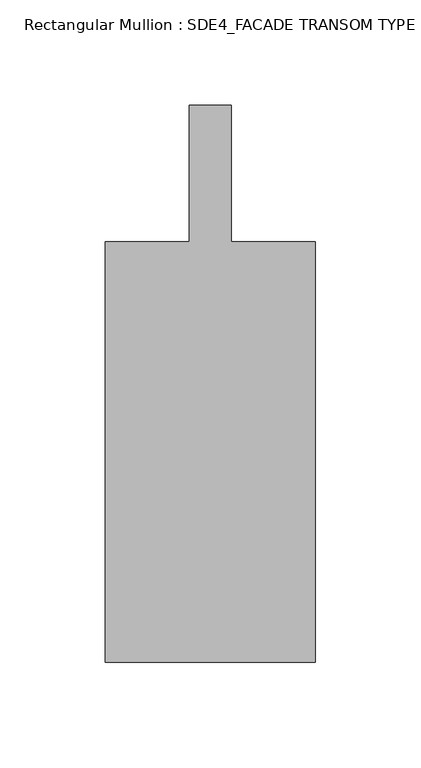
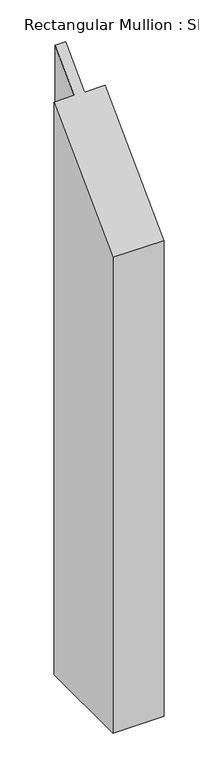
"""IFC4 building model written with IfcOpenShell, lengths in millimetres: member geometry, Rectangular Mullion : SDE4_FACADE TRANSOM TYPE 2."""

from ifc_helpers import new_model, si_unit, origin, place, context, project, spatial, faceted_brep, source, transform, mapped, element, save


def rectangular_mullion_sde4_facade_transom_type_2_c3290715(model_context):
    return source(origin(), model_context, "Body", "Brep", [
        faceted_brep([(50.0, -132.5, -1117.3997609), (-50.0, -132.5, -1117.3997609), (-50.0, 67.5, -1117.3997609), (-10.0, 67.5, -1117.3997609), (-10.0, 132.5, -1117.3997609), (10.0, 132.5, -1117.3997609), (10.0, 67.5, -1117.3997609), (50.0, 67.5, -1117.3997609), (50.0, 67.5, 67.5), (50.0, -132.5, -132.5), (10.0, 67.5, 67.5), (10.0, 132.5, 132.5), (-10.0, 132.5, 132.5), (-10.0, 67.5, 67.5), (-50.0, 67.5, 67.5), (-50.0, -132.5, -132.5)], [[[0, 1, 2, 3, 4, 5, 6, 7]], [[8, 9, 0, 7]], [[10, 8, 7, 6]], [[11, 10, 6, 5]], [[12, 11, 5, 4]], [[13, 12, 4, 3]], [[14, 13, 3, 2]], [[15, 14, 2, 1]], [[9, 15, 1, 0]], [[9, 8, 10, 11, 12, 13, 14, 15]]]),
    ])


if __name__ == "__main__":
    model = new_model("IFC4")
    model_context = context("Model", 3, world=origin())
    ifc_project = project(units=[si_unit("LENGTHUNIT", "METRE", prefix="MILLI")], contexts=[model_context])
    site = spatial("IfcSite", under=ifc_project)
    building = spatial("IfcBuilding", under=site)
    placement = place(None, origin())
    rectangular_mullion_sde4_facade_transom_type_2_shape = rectangular_mullion_sde4_facade_transom_type_2_c3290715(model_context)
    element("IfcMember", 1, ObjectType="Rectangular Mullion : SDE4_FACADE TRANSOM TYPE 2", at=placement, inside=building, context=model_context, shape_type="MappedRepresentation", body=[
        mapped(rectangular_mullion_sde4_facade_transom_type_2_shape, transform((0.0, 0.0, 0.0), x_axis=(1.0, 0.0, 0.0), y_axis=(0.0, 1.0, 0.0), z_axis=(0.0, 0.0, 1.0))),
    ])
    save(model, "model.ifc")

# Revit data of these elements
# Type "Rectangular Mullion : SDE4_FACADE TRANSOM TYPE 2"
#   built-in parameter 1007322 = 0.869423 (stored number, unit not read)
#   built-in parameter 1007321 = 0.164042 (stored number, unit not read)
#   built-in parameter 1007320 = 0.164042 (stored number, unit not read)
